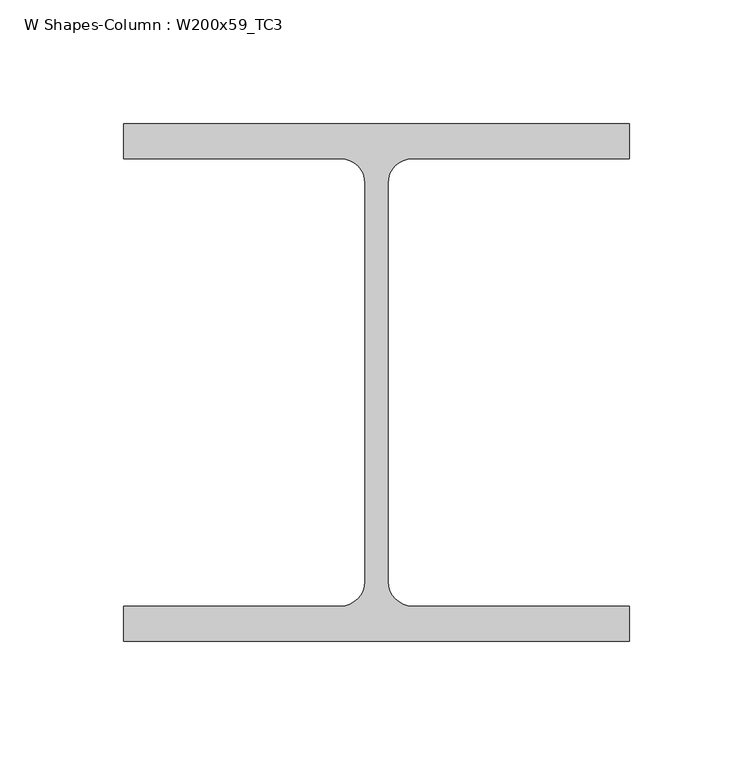
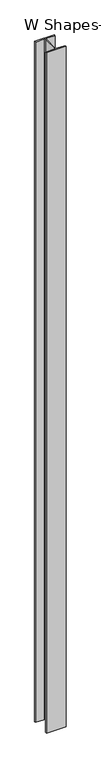
"""IFC4 building model written with IfcOpenShell, lengths in millimetres: column geometry, W Shapes-Column : W200x59_TC3."""

from ifc_helpers import new_model, si_unit, point, frame, frame_2d, origin, place, context, project, spatial, polyline, circle_curve, trimmed, segment, composite_curve, outline, extrude, source, transform, mapped, element, save


def w_shapes_column_w200x59_tc3_783e3835(model_context):
    return source(origin(), model_context, "Body", "SweptSolid", [
        extrude(outline(composite_curve([segment(polyline([(102.489, -104.775), (-102.489, -104.775), (-102.489, -90.551), (-14.5796, -90.551)]), True, "CONTINUOUS"), segment(trimmed(circle_curve(frame_2d((-14.5796, -80.5434)), 10.0076), [point((-14.5796, -90.551))], [point((-4.572, -80.5434))], True, "CARTESIAN"), True, "CONTINUOUS"), segment(polyline([(-4.572, -80.5434), (-4.572, 80.5434)]), True, "CONTINUOUS"), segment(trimmed(circle_curve(frame_2d((-14.5796, 80.5434)), 10.0076), [point((-4.572, 80.5434))], [point((-14.5796, 90.551))], True, "CARTESIAN"), True, "CONTINUOUS"), segment(polyline([(-14.5796, 90.551), (-102.489, 90.551), (-102.489, 104.775), (102.489, 104.775), (102.489, 90.551), (14.5796, 90.551)]), True, "CONTINUOUS"), segment(trimmed(circle_curve(frame_2d((14.5796, 80.5434)), 10.0076), [point((14.5796, 90.551))], [point((4.572, 80.5434))], True, "CARTESIAN"), True, "CONTINUOUS"), segment(polyline([(4.572, 80.5434), (4.572, -80.5434)]), True, "CONTINUOUS"), segment(trimmed(circle_curve(frame_2d((14.5796, -80.5434)), 10.0076), [point((4.572, -80.5434))], [point((14.5796, -90.551))], True, "CARTESIAN"), True, "CONTINUOUS"), segment(polyline([(14.5796, -90.551), (102.489, -90.551), (102.489, -104.775)]), True, "CONTINUOUS")], self_intersect=False)), frame((0.0, 0.0, 200.0), z_axis=(0.0, 0.0, 1.0), x_axis=(1.0, 0.0, 0.0)), (0.0, 0.0, 1.0), 7500.0),
    ])


if __name__ == "__main__":
    model = new_model("IFC4")
    model_context = context("Model", 3, world=origin())
    ifc_project = project(units=[si_unit("LENGTHUNIT", "METRE", prefix="MILLI")], contexts=[model_context])
    site = spatial("IfcSite", under=ifc_project)
    building = spatial("IfcBuilding", under=site)
    placement = place(None, origin())
    w_shapes_column_w200x59_tc3_shape = w_shapes_column_w200x59_tc3_783e3835(model_context)
    element("IfcColumn", 1, ObjectType="W Shapes-Column : W200x59_TC3", at=placement, inside=building, context=model_context, shape_type="MappedRepresentation", body=[
        mapped(w_shapes_column_w200x59_tc3_shape, transform((0.0, 0.0, 0.0), x_axis=(1.0, 0.0, 0.0), y_axis=(0.0, 1.0, 0.0), z_axis=(0.0, 0.0, 1.0))),
    ])
    save(model, "model.ifc")

# Revit data of these elements
# Type "W Shapes-Column : W200x59_TC3"
#   Section Name Key = "W8X40"
#   Assembly Code = "B10"
#   Width = 20.4978 cm
#   Web Thickness = 0.9144 cm
#   Web Fillet = 1.0008 cm
#   Warping Constant = 194957.0 cm⁶
#   Torsional Moment of Inertia = 46.6179 cm⁴
#   Section Area = 75.4837 cm²
#   Plastic Modulus weak axis = 303.161 cm³
#   Plastic Modulus strong axis = 652.205 cm³
#   Perimeter = 1.20396 m²/m
#   Nominal Weight = 59.5266 kgf/m
#   Moment of Inertia weak axis = 2043.70 cm⁴
#   Moment of Inertia strong axis = 6076.98 cm⁴
#   Height = 20.955 cm
#   Flange Thickness = 1.4224 cm
#   Elastic Modulus weak axis = 199.922 cm³
#   Elastic Modulus strong axis = 581.741 cm³
#   Clear Web Height = 14.605 cm
#   Centroid Vertical = 10.4775 cm
#   Centroid Horizontal = 10.2489 cm
#   Bolt Spacing = 13.97 cm
#   Structural Material [instance default] = Steel ASTM A992
#   Principal Axes Angle = 0
# Element 1 (IfcColumn, "W Shapes-Column : W200x59_TC3")
#   Structural Material = none
# Materials
#   "Steel ASTM A992": class "Metal", colour RGB 199 199 199, transparency 0, Description = "Structural steel 50ksi", Cost = 0
